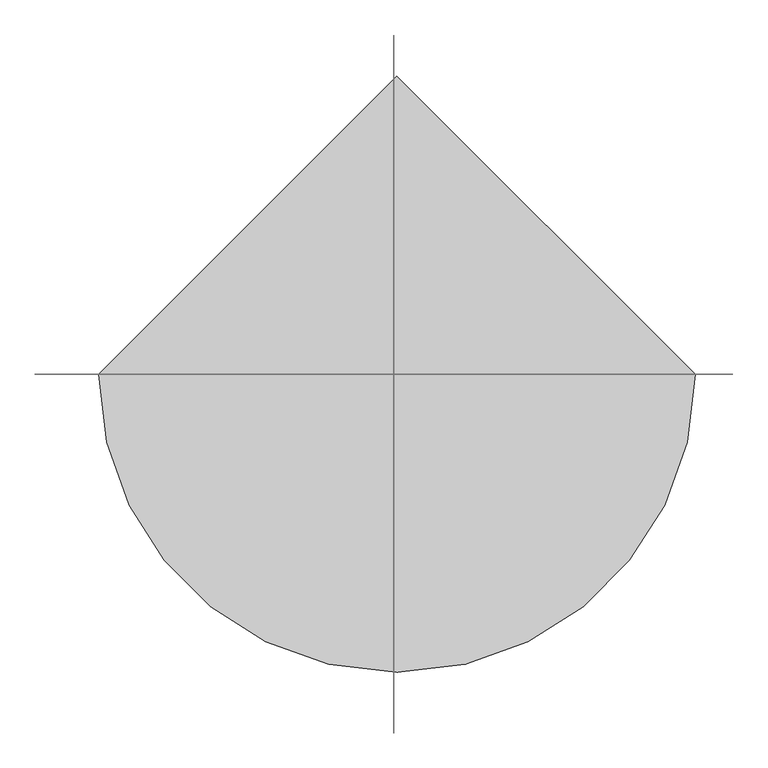
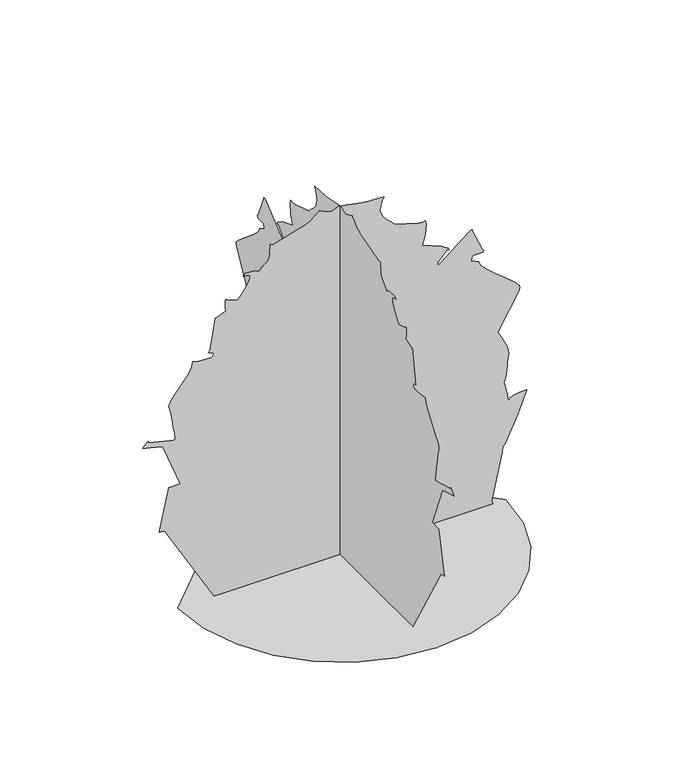
"""IFC4 building model written with IfcOpenShell, lengths in millimetres: proxy geometry, fraser photina 26748 : fraser photina 26748."""

from ifc_helpers import new_model, si_unit, origin, place, context, project, spatial, triangles, source, transform, mapped, element, save


def entourage_08a53f53(model_context):
    return source(origin(), model_context, "Body", "Tessellation", [
        triangles([(-943.2294903, 0.0, 1.5e-05), (-918.294239, -216.1259976, 1.5e-05), (-847.2781523, -414.6029998, 1.5e-05), (-735.8657667, -589.7441626, 1.5e-05), (-589.7441626, -735.8657667, 1.5e-05), (-414.6029998, -847.2781523, 1.5e-05), (-216.1259976, -918.294239, 1.5e-05), (4.12e-05, -943.2294903, 1.5e-05), (216.1259976, -918.294239, 1.5e-05), (414.6029998, -847.2781523, 1.5e-05), (589.7441626, -735.8657667, 1.5e-05), (735.8657667, -589.7441626, 1.5e-05), (847.2781523, -414.6029998, 1.5e-05), (918.294239, -216.1257432, 1.5e-05), (943.2294903, 8.25e-05, 1.5e-05), (-0.0001237, 943.2294903, 1.5e-05), (-1017.298661, 9.78e-05, 493.3025928), (-1050.3238255, 9.75e-05, 498.806799), (-995.2792929, 8.24e-05, 752.007514), (-929.2264206, 8.24e-05, 752.007514), (-1028.3070734, 6.73e-05, 1005.2081926), (-1035.1219191, 6.68e-05, 1013.229578), (-1132.4499172, 6.55e-05, 1039.4627878), (-1145.9932766, 6.52e-05, 1042.6555435), (-1143.897765, 6.5e-05, 1043.740143), (-1116.9076246, 6.56e-05, 1072.2695063), (-1112.8918814, 6.54e-05, 1074.5250372), (-1112.386389, 6.49e-05, 1072.3330198), (-1113.4837057, 6.4e-05, 1065.2819241), (-1110.8725279, 6.37e-05, 1065.7568951), (-962.2541285, 6.6e-05, 1027.2275608), (-959.3585203, 6.54e-05, 1037.0574114), (-962.0509432, 6.36e-05, 1067.5907948), (-968.5025843, 6.1e-05, 1110.7303127), (-976.8820147, 5.82e-05, 1158.3783491), (-985.3580235, 5.55e-05, 1202.4372877), (-992.1017979, 5.36e-05, 1234.8122738), (-995.2792929, 5.28e-05, 1247.403075), (-986.4756878, 5.16e-05, 1267.7612801), (-965.6526855, 4.99e-05, 1296.7147453), (-937.8522749, 4.78e-05, 1331.3274582), (-908.1113577, 4.56e-05, 1368.6580284), (-881.4767916, 4.34e-05, 1405.7700073), (-862.9830076, 4.14e-05, 1439.7222954), (-857.6693058, 3.97e-05, 1467.5761185), (-842.1752661, 3.99e-05, 1463.9083191), (-822.794981, 4.01e-05, 1460.9593712), (-801.8145029, 4.02e-05, 1458.7164848), (-781.5147972, 4.03e-05, 1457.1671608), (-764.1868578, 4.04e-05, 1456.3035507), (-752.1141935, 4.04e-05, 1456.1079231), (-747.5827841, 4.04e-05, 1456.5676334), (-741.99984, 4e-05, 1462.5113113), (-738.4590677, 3.97e-05, 1468.5716972), (-737.3237446, 3.93e-05, 1474.439217), (-738.9543863, 3.9e-05, 1479.7909252), (-743.7194298, 3.87e-05, 1484.314777), (-751.9769926, 3.85e-05, 1487.6878269), (-764.095439, 3.84e-05, 1489.595414), (-756.9731993, 3.77e-05, 1509.6183197), (-737.1611818, 3.35e-05, 1632.1888905), (-732.0100428, 3.15e-05, 1668.3611012), (-728.0501827, 2.92e-05, 1689.4330708), (-725.566032, 2.66e-05, 1687.7516327), (-663.5568083, 2.53e-05, 1709.8014496), (-665.0173296, 2.53e-05, 1709.7709282), (-669.6604328, 2.58e-05, 1729.964027), (-671.5806644, 2.5e-05, 1762.5217781), (-670.2167215, 2.41e-05, 1773.4209675), (-668.2151722, 2.31e-05, 1779.758226), (-666.254318, 2.21e-05, 1780.802203), (-665.0173296, 2.13e-05, 1775.821257), (-607.43785, 2.25e-05, 1755.9864212), (-604.4685908, 2.27e-05, 1753.8044323), (-600.5518968, 2.28e-05, 1751.8969906), (-587.3667277, 2.2e-05, 1765.1964695), (-550.3892973, 1.89e-05, 1816.9186031), (-535.197492, 1.72e-05, 1845.0872326), (-527.9381604, 1.59e-05, 1867.9574936), (-532.911476, 1.51e-05, 1880.4061523), (-566.5157839, 1.47e-05, 1888.5595791), (-566.9450455, 1.45e-05, 1889.3215965), (-559.7949368, 1.4e-05, 1895.0619438), (-554.9308079, 1.38e-05, 1902.4229771), (-498.5731287, 1.36e-05, 1897.6171658), (-472.3653171, 1.48e-05, 1885.9103222), (-468.1895545, 1.45e-05, 1891.508527), (-465.0780438, 1.42e-05, 1896.0652256), (-462.4415042, 1.4e-05, 1899.8726967), (-459.6881475, 1.38e-05, 1903.2204575), (-456.2311638, 1.36e-05, 1906.403112), (-451.4788376, 1.34e-05, 1909.7101776), (-444.841779, 1.31e-05, 1913.4313168), (-433.2390352, 1.26e-05, 1921.9479481), (-424.2626209, 1.19e-05, 1934.5997921), (-417.711967, 1.09e-05, 1950.3478134), (-413.388866, 9.9e-06, 1968.1557381), (-411.8166146, 6.6e-06, 2023.5203819), (-391.9588151, 6.7e-06, 2021.3155746), (-197.9733084, 3.3e-06, 2078.1025154), (-186.1363674, 3e-06, 2084.0665409), (-180.1988482, 2.9e-06, 2085.2705372), (-140.4007233, 8e-07, 2119.9339737), (-133.6608186, 3e-07, 2128.3591862), (-131.092616, 0.0, 2133.606831), (-82.7930932, 1.4e-06, 2110.2082592), (-69.1275892, 1.6e-06, 2106.3118401), (-54.9624745, 1.7e-06, 2106.3018116), (-39.2652223, 1.3e-06, 2111.343655), (-21.0049792, 7e-07, 2122.5984913), (133.5632773, 3.1e-06, 2091.986261), (241.2631805, 5.2e-06, 2088.6588478), (244.7076832, 4.8e-06, 2084.5846779), (232.1963648, 3.6e-06, 2073.0580559), (218.8971402, 7.3e-06, 2011.3105167), (218.7703856, 7.6e-06, 2007.0179008), (221.1872076, 7.6e-06, 2007.0052563), (229.3777142, 9e-06, 1983.1850533), (238.1326122, 1e-05, 1966.0475819), (247.6764519, 1.08e-05, 1953.3602749), (258.2350007, 1.14e-05, 1942.8878036), (270.0333358, 1.2e-05, 1932.3976009), (283.2972609, 1.28e-05, 1919.6543381), (298.2477473, 1.38e-05, 1902.4229771), (308.9386645, 1.42e-05, 1896.5884495), (440.1326188, 1.65e-05, 1856.8094822), (466.8636543, 1.67e-05, 1853.9442501), (479.893891, 1.64e-05, 1858.3868568), (485.2711063, 1.76e-05, 1839.3265377), (481.2756743, 2.16e-05, 1771.8232452), (463.3813087, 2.5e-05, 1715.275098), (568.0042468, 2.51e-05, 1673.2583313), (612.6067932, 2.65e-05, 1643.8678288), (618.044906, 2.74e-05, 1636.0167091), (615.253434, 2.85e-05, 1633.8501263), (606.4929949, 2.96e-05, 1638.2138134), (556.810417, 3.27e-05, 1586.1207722), (551.4484623, 3.28e-05, 1583.1693535), (551.4484623, 3.41e-05, 1561.1525288), (566.759628, 3.37e-05, 1568.6607914), (732.9472675, 2.77e-05, 1703.5910728), (742.9422243, 2.82e-05, 1708.7574726), (748.062842, 2.8e-05, 1710.1062275), (749.7976925, 2.74e-05, 1708.9834763), (749.6376732, 2.66e-05, 1706.7381191), (749.078841, 2.59e-05, 1704.7138241), (749.6072245, 2.56e-05, 1704.2641422), (807.1231178, 3.31e-05, 1570.456612), (815.6600967, 3.41e-05, 1561.1525288), (811.6189917, 3.43e-05, 1557.7336967), (811.8018293, 3.45e-05, 1554.8049511), (812.5942955, 3.46e-05, 1552.4427406), (810.3870174, 3.47e-05, 1550.7181366), (749.6072245, 3.48e-05, 1550.141573), (744.1029819, 3.64e-05, 1522.6205784), (788.1391022, 3.78e-05, 1500.6037537), (797.9689528, 3.92e-05, 1476.5829815), (834.161511, 4.14e-05, 1439.2574982), (885.6957201, 4.41e-05, 1394.6499012), (941.5479795, 4.68e-05, 1348.787439), (990.7022467, 4.93e-05, 1307.6951797), (1022.1348484, 5.11e-05, 1277.3954304), (1024.8272713, 5.19e-05, 1263.9157299), (1020.029163, 5.3e-05, 1245.6200443), (898.2256239, 6.56e-05, 1032.7317307), (908.5380758, 6.67e-05, 1015.3276331), (921.499712, 6.81e-05, 991.0299156), (935.1929169, 6.98e-05, 962.5767105), (947.6872124, 7.16e-05, 932.7138531), (957.0649103, 7.33e-05, 904.1844898), (961.4032356, 7.48e-05, 879.7318399), (958.7743263, 7.58e-05, 862.0965065), (953.9432259, 7.65e-05, 850.5903048), (951.748665, 7.75e-05, 833.3233355), (950.7910927, 7.88e-05, 811.8043728), (949.6633272, 8.03e-05, 787.5498213), (946.9658175, 8.18e-05, 762.0684551), (941.2965414, 8.33e-05, 736.8741354), (931.2533318, 8.47e-05, 713.4781071), (936.3003347, 8.52e-05, 703.8692459), (941.4159382, 8.63e-05, 685.4440624), (946.3333706, 8.77e-05, 661.9489849), (950.7910927, 8.92e-05, 637.1432316), (954.5274199, 9.06e-05, 614.778463), (957.2757259, 9.15e-05, 598.606267), (958.7743263, 9.19e-05, 592.3807022), (967.1106634, 9.1e-05, 606.6402969), (982.477676, 9.04e-05, 616.5666533), (1022.7164989, 8.99e-05, 626.1856882), (1056.303039, 8.98e-05, 626.7724257), (1063.3566055, 8.99e-05, 625.4084101), (1011.388048, 9.77e-05, 494.3947864), (939.8487373, 0.0001067, 343.3938652), (925.7491619, 0.0001076, 328.1715749), (924.4791086, 0.0001095, 297.0691855), (862.2286205, 0.000126, 22.7715025), (867.6845375, 0.0001272, 0.0001027), (-733.7118284, 0.0001272, 0.0001027), (-9.9961263, -1007.3011608, 493.3025928), (-9.9961263, -1040.3263979, 498.806799), (-9.9961263, -985.2844088, 752.007514), (-9.9961263, -919.2314638, 752.007514), (-9.9961002, -1018.3095732, 1005.2081926), (-9.9961002, -1025.1244188, 1013.229578), (-9.9961002, -1122.452417, 1039.4627878), (-9.9961002, -1135.9957764, 1042.6555435), (-9.9961002, -1133.9028082, 1043.740143), (-9.9961002, -1106.9126678, 1072.2695063), (-9.9961002, -1102.8969246, 1074.5250372), (-9.9961002, -1102.3889614, 1072.3330198), (-9.9961002, -1103.4862055, 1065.2819241), (-9.9961002, -1100.8751003, 1065.7568951), (-9.9961002, -952.2591717, 1027.2275608), (-9.9961002, -949.3610928, 1037.0574114), (-9.9961002, -952.053443, 1067.5907948), (-9.9961002, -958.505084, 1110.7303127), (-9.9961002, -966.8845871, 1158.3783491), (-9.9961002, -975.3631393, 1202.4372877), (-9.9961002, -982.1042976, 1234.8122738), (-9.9961002, -985.2844088, 1247.403075), (-9.9961002, -976.4781876, 1267.7612801), (-9.9961002, -955.6551853, 1296.7147453), (-9.9961002, -927.8547747, 1331.3274582), (-9.9961002, -898.1164009, 1368.6580284), (-9.9961002, -871.4818348, 1405.7700073), (-9.9961002, -852.9855074, 1439.7222954), (-9.9961002, -847.674349, 1467.5761185), (-9.9961002, -832.1803093, 1463.9083191), (-9.9961002, -812.8000969, 1460.9593712), (-9.9961002, -791.8170753, 1458.7164848), (-9.9961002, -771.5198404, 1457.1671608), (-9.9961002, -754.191901, 1456.3035507), (-9.9961002, -742.1192368, 1456.1079231), (-9.9961002, -737.5879, 1456.5676334), (-9.9961002, -732.0049559, 1462.5113113), (-9.9961002, -728.4641836, 1468.5716972), (-9.9961002, -727.3262444, 1474.439217), (-9.9961002, -728.9569588, 1479.7909252), (-9.9961002, -733.7220022, 1484.314777), (-9.9961002, -741.9821085, 1487.6878269), (-9.9961002, -754.1004822, 1489.595414), (-9.9961002, -746.9783152, 1509.6183197), (-9.9961002, -727.1662251, 1632.1888905), (-9.9961002, -722.015086, 1668.3611012), (-9.9961002, -718.0552259, 1689.4330708), (-9.9961002, -715.5685318, 1687.7516327), (-9.9961002, -653.5618515, 1709.8014496), (-9.9961002, -655.0223728, 1709.7709282), (-9.9961002, -659.665476, 1729.964027), (-9.9961002, -661.5832369, 1762.5217781), (-9.9961002, -660.2192213, 1773.4209675), (-9.9961002, -658.217672, 1779.758226), (-9.9961002, -656.2593613, 1780.802203), (-9.9961002, -655.0223728, 1775.821257), (-9.9961002, -597.4429296, 1755.9864212), (-9.9961002, -594.4736704, 1753.8044323), (-9.9961002, -590.5544329, 1751.8969906), (-9.9961002, -577.3692638, 1765.1964695), (-9.9961002, -540.3917971, 1816.9186031), (-9.9961002, -525.2025716, 1845.0872326), (-9.9961002, -517.9432036, 1867.9574936), (-9.9961002, -522.9165556, 1880.4061523), (-9.9961002, -556.5208634, 1888.5595791), (-9.9960752, -556.950125, 1889.3215965), (-9.9960752, -549.8000164, 1895.0619438), (-9.9960752, -544.933344, 1902.4229771), (-9.9961002, -488.5781719, 1897.6171658), (-9.9961002, -462.3678532, 1885.9103222), (-9.9961002, -458.1945977, 1891.508527), (-9.9961002, -455.0830871, 1896.0652256), (-9.9961002, -452.4440403, 1899.8726967), (-9.9961002, -449.6906473, 1903.2204575), (-9.9961002, -446.2336999, 1906.403112), (-9.9961002, -441.4813374, 1909.7101776), (-9.9961002, -434.8468586, 1913.4313168), (-9.9961002, -423.2440784, 1921.9479481), (-9.9961002, -414.265157, 1934.5997921), (-9.9961002, -407.7144668, 1950.3478134), (-9.9960752, -403.3914021, 1968.1557381), (-9.9960752, -401.8191144, 2023.5203819), (-9.9960752, -381.9613512, 2021.3155746), (-9.9960752, -187.9771162, 2078.1025154), (-9.9960752, -176.1404114, 2084.0665409), (-9.9960752, -170.2028923, 2085.2705372), (-9.9960752, -130.4047764, 2119.9339737), (-9.9960752, -123.6646173, 2128.3591862), (-9.9960752, -121.0966691, 2133.606831), (-9.9961002, -72.7968874, 2110.2082592), (-9.9961002, -59.131388, 2106.3118401), (-9.9961002, -44.9665276, 2106.3018116), (-9.9961002, -29.269021, 2111.343655), (-9.9961002, -11.0088779, 2122.5984913), (-9.9961002, 143.5592242, 2091.986261), (-9.9961002, 251.2593909, 2088.6588478), (-9.9961002, 254.7044023, 2084.5846779), (-9.9961002, 242.1923208, 2073.0580559), (-9.9961002, 228.8933324, 2011.3105167), (-9.9961002, 228.7663416, 2007.0179008), (-9.9961002, 231.1831635, 2007.0052563), (-9.9961002, 239.3739245, 1983.1850533), (-9.9961002, 248.1285682, 1966.0475819), (-9.9961002, 257.6736614, 1953.3602749), (-9.9961002, 268.2324828, 1942.8878036), (-9.9961002, 280.0282744, 1932.3976009), (-9.9961002, 293.2921995, 1919.6543381), (-9.9961002, 308.2452112, 1902.4229771), (-9.9961002, 318.9361284, 1896.5884495), (-9.9961002, 450.1300827, 1856.8094822), (-9.9961002, 476.8585748, 1853.9442501), (-9.9961002, 489.8888114, 1858.3868568), (-9.9961002, 495.2660268, 1839.3265377), (-9.9961002, 491.2731382, 1771.8232452), (-9.9961002, 473.3762292, 1715.275098), (-9.9961002, 578.0017107, 1673.2583313), (-9.9961002, 622.6016773, 1643.8678288), (-9.9961002, 628.0398628, 1636.0167091), (-9.9961002, 625.2509342, 1633.8501263), (-9.9961002, 616.4904224, 1638.2138134), (-9.9961002, 566.8053374, 1586.1207722), (-9.9961002, 561.4459262, 1583.1693535), (-9.9961263, 561.4459262, 1561.1525288), (-9.9961263, 576.7545485, 1568.6607914), (-9.9961263, 742.9422243, 1703.5910728), (-9.9961263, 752.9397245, 1708.7574726), (-9.9961263, 758.0603422, 1710.1062275), (-9.9961263, 759.7926493, 1708.9834763), (-9.9961263, 759.6351734, 1706.7381191), (-9.9961002, 759.0737978, 1704.7138241), (-9.9961002, 759.604652, 1704.2641422), (-9.9961263, 817.1206181, 1570.456612), (-9.9961263, 825.657597, 1561.1525288), (-9.9961263, 821.6138758, 1557.7336967), (-9.9961263, 821.7967861, 1554.8049511), (-9.9961263, 822.5917957, 1552.4427406), (-9.9961263, 820.3819742, 1550.7181366), (-9.9961263, 759.604652, 1550.141573), (-9.9961263, 754.0979387, 1522.6205784), (-9.9961263, 798.134059, 1500.6037537), (-9.9961263, 807.966453, 1476.5829815), (-9.9961263, 844.1590113, 1439.2574982), (-9.9961263, 895.6906769, 1394.6499012), (-9.9961263, 951.5454798, 1348.787439), (-9.9961263, 1000.6971308, 1307.6951797), (-9.9961263, 1032.132276, 1277.3954304), (-9.9961263, 1034.8221554, 1263.9157299), (-9.9961263, 1030.0241198, 1245.6200443), (-9.9961263, 908.2230515, 1032.7317307), (-9.9961263, 918.5329599, 1015.3276331), (-9.9961263, 931.4972122, 991.0299156), (-9.9961263, 945.187801, 962.5767105), (-9.9961513, 957.6846399, 932.7138531), (-9.9961513, 967.0624105, 904.1844898), (-9.9961513, 971.3981924, 879.7318399), (-9.9961513, 968.7692831, 862.0965065), (-9.9961513, 963.9407261, 850.5903048), (-9.9961513, 961.7461653, 833.3233355), (-9.9961513, 960.7860495, 811.8043728), (-9.9961513, 959.6607548, 787.5498213), (-9.9961513, 956.9633177, 762.0684551), (-9.9961513, 951.293969, 736.8741354), (-9.9961513, 941.2482885, 713.4781071), (-9.9961513, 946.2952915, 703.8692459), (-9.9961513, 951.4108223, 685.4440624), (-9.9961513, 956.3283274, 661.9489849), (-9.9961513, 960.7885202, 637.1432316), (-9.9961513, 964.5223766, 614.778463), (-9.9961513, 967.2706827, 598.606267), (-9.9961513, 968.7692831, 592.3807022), (-9.9961513, 977.1055475, 606.6402969), (-9.9961513, 992.4751762, 616.5666533), (-9.9961513, 1032.7114557, 626.1856882), (-9.9961513, 1066.3004665, 626.7724257), (-9.9961513, 1073.3541058, 625.4084101), (-9.9961513, 1021.3855482, 494.3947864), (-9.9961513, 949.8436941, 343.3938652), (-9.9961513, 935.744046, 328.1715749), (-9.9961513, 934.4766088, 297.0691855), (-9.9961763, 872.2235773, 22.7714026), (-9.9961763, 877.6794943, 0.0), (-9.9961513, -723.7168716, 4.77e-05)], [[15, 16, 1], [14, 15, 1], [14, 1, 2], [13, 14, 2], [13, 2, 3], [13, 3, 4], [12, 13, 4], [11, 12, 4], [11, 4, 5], [11, 5, 6], [11, 6, 7], [11, 7, 8], [11, 8, 9], [11, 9, 10], [23, 24, 25], [62, 63, 64], [26, 27, 28], [70, 71, 72], [69, 70, 72], [196, 197, 198], [58, 59, 60], [97, 98, 99], [190, 191, 192], [127, 128, 129], [17, 18, 19], [44, 45, 46], [148, 149, 150], [25, 26, 28], [25, 28, 29], [23, 25, 29], [104, 105, 106], [23, 29, 30], [23, 30, 31], [22, 23, 31], [21, 22, 31], [20, 21, 31], [112, 113, 114], [111, 112, 114], [133, 134, 135], [133, 135, 136], [132, 133, 136], [81, 82, 83], [80, 81, 83], [17, 19, 20], [65, 66, 67], [80, 83, 84], [80, 84, 85], [189, 190, 192], [79, 80, 85], [116, 117, 118], [151, 152, 153], [195, 196, 198], [194, 195, 198], [194, 198, 17], [194, 17, 20], [194, 20, 31], [194, 31, 32], [188, 189, 192], [187, 188, 192], [186, 187, 192], [193, 194, 32], [192, 193, 32], [186, 192, 32], [185, 186, 32], [184, 185, 32], [183, 184, 32], [182, 183, 32], [181, 182, 32], [180, 181, 32], [179, 180, 32], [178, 179, 32], [177, 178, 32], [176, 177, 32], [175, 176, 32], [174, 175, 32], [173, 174, 32], [173, 32, 33], [173, 33, 34], [172, 173, 34], [171, 172, 34], [170, 171, 34], [169, 170, 34], [168, 169, 34], [167, 168, 34], [166, 167, 34], [165, 166, 34], [165, 34, 35], [165, 35, 36], [165, 36, 37], [165, 37, 38], [165, 38, 39], [165, 39, 40], [165, 40, 41], [165, 41, 42], [165, 42, 43], [165, 43, 44], [165, 44, 46], [165, 46, 47], [165, 47, 48], [165, 48, 49], [165, 49, 50], [165, 50, 51], [165, 51, 52], [165, 52, 53], [165, 53, 54], [165, 54, 55], [164, 165, 55], [163, 164, 55], [162, 163, 55], [161, 162, 55], [160, 161, 55], [159, 160, 55], [158, 159, 55], [157, 158, 55], [156, 157, 55], [155, 156, 55], [154, 155, 55], [154, 55, 56], [150, 151, 153], [148, 150, 153], [143, 144, 145], [142, 143, 145], [142, 145, 146], [141, 142, 146], [103, 104, 106], [132, 136, 137], [132, 137, 138], [68, 69, 72], [131, 132, 138], [148, 153, 154], [57, 58, 60], [67, 68, 72], [65, 67, 72], [65, 72, 73], [65, 73, 74], [65, 74, 75], [111, 114, 115], [78, 79, 85], [78, 85, 86], [111, 115, 116], [126, 127, 129], [154, 56, 57], [154, 57, 60], [154, 60, 61], [126, 129, 130], [126, 130, 131], [109, 110, 111], [141, 146, 147], [141, 147, 148], [141, 148, 154], [140, 141, 154], [62, 64, 65], [125, 126, 131], [111, 116, 118], [61, 62, 65], [131, 138, 139], [139, 140, 154], [139, 154, 61], [139, 61, 65], [139, 65, 75], [131, 139, 75], [131, 75, 76], [125, 131, 76], [124, 125, 76], [124, 76, 77], [123, 124, 77], [122, 123, 77], [121, 122, 77], [121, 77, 78], [121, 78, 86], [121, 86, 87], [120, 121, 87], [120, 87, 88], [120, 88, 89], [120, 89, 90], [120, 90, 91], [120, 91, 92], [120, 92, 93], [120, 93, 94], [120, 94, 95], [119, 120, 95], [119, 95, 96], [118, 119, 96], [111, 118, 96], [109, 111, 96], [108, 109, 96], [107, 108, 96], [106, 107, 96], [106, 96, 97], [102, 103, 106], [102, 106, 97], [101, 102, 97], [100, 101, 97], [100, 97, 99], [205, 206, 207], [244, 245, 246], [208, 209, 210], [252, 253, 254], [251, 252, 254], [378, 379, 380], [240, 241, 242], [279, 280, 281], [372, 373, 374], [309, 310, 311], [199, 200, 201], [226, 227, 228], [330, 331, 332], [207, 208, 210], [207, 210, 211], [205, 207, 211], [286, 287, 288], [205, 211, 212], [205, 212, 213], [204, 205, 213], [203, 204, 213], [202, 203, 213], [294, 295, 296], [293, 294, 296], [315, 316, 317], [315, 317, 318], [314, 315, 318], [263, 264, 265], [262, 263, 265], [199, 201, 202], [247, 248, 249], [262, 265, 266], [262, 266, 267], [371, 372, 374], [261, 262, 267], [298, 299, 300], [333, 334, 335], [377, 378, 380], [376, 377, 380], [376, 380, 199], [376, 199, 202], [376, 202, 213], [376, 213, 214], [370, 371, 374], [369, 370, 374], [368, 369, 374], [375, 376, 214], [374, 375, 214], [368, 374, 214], [367, 368, 214], [366, 367, 214], [365, 366, 214], [364, 365, 214], [363, 364, 214], [362, 363, 214], [361, 362, 214], [360, 361, 214], [359, 360, 214], [358, 359, 214], [357, 358, 214], [356, 357, 214], [355, 356, 214], [355, 214, 215], [355, 215, 216], [354, 355, 216], [353, 354, 216], [352, 353, 216], [351, 352, 216], [350, 351, 216], [349, 350, 216], [348, 349, 216], [347, 348, 216], [347, 216, 217], [347, 217, 218], [347, 218, 219], [347, 219, 220], [347, 220, 221], [347, 221, 222], [347, 222, 223], [347, 223, 224], [347, 224, 225], [347, 225, 226], [347, 226, 228], [347, 228, 229], [347, 229, 230], [347, 230, 231], [347, 231, 232], [347, 232, 233], [347, 233, 234], [347, 234, 235], [347, 235, 236], [347, 236, 237], [346, 347, 237], [345, 346, 237], [344, 345, 237], [343, 344, 237], [342, 343, 237], [341, 342, 237], [340, 341, 237], [339, 340, 237], [338, 339, 237], [337, 338, 237], [336, 337, 237], [336, 237, 238], [332, 333, 335], [330, 332, 335], [325, 326, 327], [324, 325, 327], [324, 327, 328], [323, 324, 328], [285, 286, 288], [314, 318, 319], [314, 319, 320], [250, 251, 254], [313, 314, 320], [330, 335, 336], [239, 240, 242], [249, 250, 254], [247, 249, 254], [247, 254, 255], [247, 255, 256], [247, 256, 257], [293, 296, 297], [260, 261, 267], [260, 267, 268], [293, 297, 298], [308, 309, 311], [336, 238, 239], [336, 239, 242], [336, 242, 243], [308, 311, 312], [308, 312, 313], [291, 292, 293], [323, 328, 329], [323, 329, 330], [323, 330, 336], [322, 323, 336], [244, 246, 247], [307, 308, 313], [293, 298, 300], [243, 244, 247], [313, 320, 321], [321, 322, 336], [321, 336, 243], [321, 243, 247], [321, 247, 257], [313, 321, 257], [313, 257, 258], [307, 313, 258], [306, 307, 258], [306, 258, 259], [305, 306, 259], [304, 305, 259], [303, 304, 259], [303, 259, 260], [303, 260, 268], [303, 268, 269], [302, 303, 269], [302, 269, 270], [302, 270, 271], [302, 271, 272], [302, 272, 273], [302, 273, 274], [302, 274, 275], [302, 275, 276], [302, 276, 277], [301, 302, 277], [301, 277, 278], [300, 301, 278], [293, 300, 278], [291, 293, 278], [290, 291, 278], [289, 290, 278], [288, 289, 278], [288, 278, 279], [284, 285, 288], [284, 288, 279], [283, 284, 279], [282, 283, 279], [282, 279, 281]], closed=False),
    ])


if __name__ == "__main__":
    model = new_model("IFC4")
    model_context = context("Model", 3, world=origin())
    ifc_project = project(units=[si_unit("LENGTHUNIT", "METRE", prefix="MILLI")], contexts=[model_context])
    site = spatial("IfcSite", under=ifc_project)
    building = spatial("IfcBuilding", under=site)
    placement = place(None, origin())
    entourage_shape = entourage_08a53f53(model_context)
    element("IfcBuildingElementProxy", 1, Name="fraser photina 26748 : fraser photina 26748", ObjectType="fraser photina 26748 : fraser photina 26748", at=placement, inside=building, context=model_context, shape_type="MappedRepresentation", body=[
        mapped(entourage_shape, transform((0.0, 0.0, 0.0), x_axis=(1.0, 0.0, 0.0), y_axis=(0.0, 1.0, 0.0), z_axis=(0.0, 0.0, 1.0))),
    ])
    save(model, "model.ifc")

# Revit data of these elements
# Type "fraser photina 26748 : fraser photina 26748"
#   built-in parameter 1005195 = "RPC-16-G1TJ-U580-XE0H-6000-ST1L-LVER-AU"
#   Height = 0
